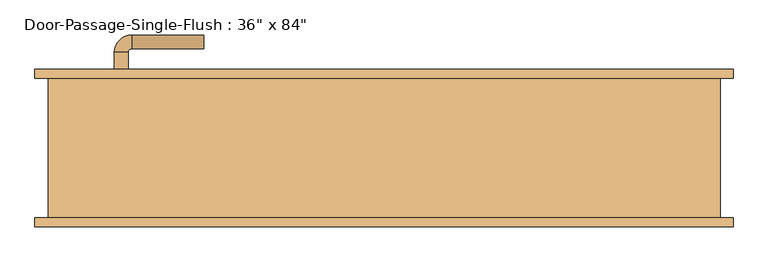
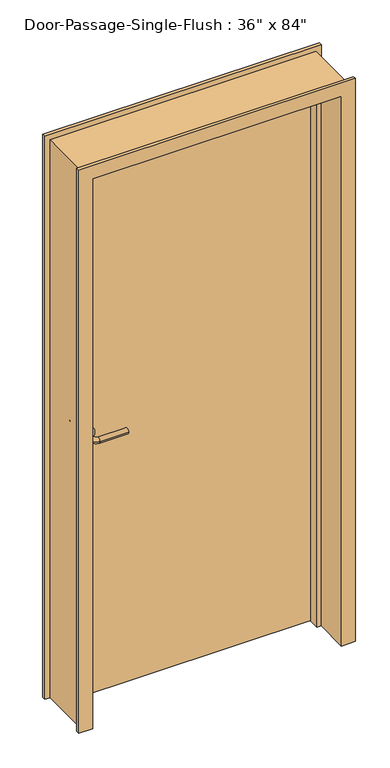
"""IFC4 building model written with IfcOpenShell, lengths in millimetres: door geometry."""

from ifc_helpers import new_model, si_unit, point, frame, frame_2d, origin, origin_with_axes, place, context, project, spatial, polyline, circle_curve, ellipse_curve, trimmed, segment, composite_curve, outline, extrude, faceted_brep, source, transform, mapped, element, save
from ifc_brep_helpers import plane_surface, cylinder_surface, revolved_surface, advanced_brep


def door_7e479f3f(model_context):
    return source(origin(), model_context, "Body", "SolidModel", [
        advanced_brep(
        [(-392.190625, 55.5, 1016.0), (-372.190625, 55.5, 1016.0), (-372.190625, 25.5, 1016.0), (-392.190625, 25.5, 1016.0), (-367.190625, 20.5, 1016.0), (-367.190625, 0.5, 1016.0), (-262.190625, 0.5, 1016.0), (-262.190625, 20.5, 1016.0)],
        [
            (0, 1, circle_curve(frame((-382.190625, 55.5, 1016.0), z_axis=(0.0, 1.0, 0.0), x_axis=(1.0, 0.0, 0.0)), 10.0)),
            (1, 0, circle_curve(frame((-382.190625, 55.5, 1016.0), z_axis=(0.0, 1.0, 0.0), x_axis=(1.0, 0.0, 0.0)), 10.0)),
            (1, 2),
            (2, 3, circle_curve(frame((-382.190625, 25.5, 1016.0), z_axis=(0.0, 1.0, 0.0), x_axis=(1.0, 0.0, 0.0)), 10.0)),
            (3, 0),
            (3, 2, circle_curve(frame((-382.190625, 25.5, 1016.0), z_axis=(0.0, 1.0, 0.0), x_axis=(1.0, 0.0, 0.0)), 10.0)),
            (4, 5, circle_curve(frame((-367.190625, 10.5, 1016.0), z_axis=(-1.0, 0.0, 0.0), x_axis=(0.0, 1.0, 0.0)), 10.0)),
            (5, 3, circle_curve(frame((-367.190625, 25.5, 1016.0), z_axis=(0.0, 0.0, -1.0), x_axis=(-1.0, 0.0, 0.0)), 25.0)),
            (2, 4, circle_curve(frame((-367.190625, 25.5, 1016.0), z_axis=(0.0, 0.0, 1.0), x_axis=(-1.0, 0.0, 0.0)), 5.0)),
            (5, 4, circle_curve(frame((-367.190625, 10.5, 1016.0), z_axis=(-1.0, 0.0, 0.0), x_axis=(0.0, 1.0, 0.0)), 10.0)),
            (6, 7, circle_curve(frame((-262.190625, 10.5, 1016.0), z_axis=(1.0, 0.0, 0.0), x_axis=(0.0, 1.0, 0.0)), 10.0)),
            (7, 6, circle_curve(frame((-262.190625, 10.5, 1016.0), z_axis=(1.0, 0.0, 0.0), x_axis=(0.0, 1.0, 0.0)), 10.0)),
            (4, 7),
            (6, 5),
        ],
        [
            plane_surface(frame((-382.190625, 55.5, 1016.0), z_axis=(0.0, 1.0, 0.0), x_axis=(0.0, 0.0, 1.0))),
            cylinder_surface(frame((-382.190625, 55.5, 1016.0), z_axis=(0.0, 1.0, 0.0), x_axis=(1.0, 0.0, 0.0)), 10.0),
            revolved_surface(trimmed(ellipse_curve(frame((-382.190625, 25.5, 1016.0), z_axis=(0.0, -1.0, 0.0), x_axis=(1.0, 0.0, 0.0)), 10.0, 10.0), [point((-392.190625, 25.5, 1016.0))], [point((-372.190625, 25.5, 1016.0))], True, "CARTESIAN"), (-367.190625, 25.5, 1016.0), (0.0, 0.0, -1.0)),
            revolved_surface(trimmed(ellipse_curve(frame((-382.190625, 25.5, 1016.0), z_axis=(0.0, -1.0, 0.0), x_axis=(1.0, 0.0, 0.0)), 10.0, 10.0), [point((-372.190625, 25.5, 1016.0))], [point((-392.190625, 25.5, 1016.0))], True, "CARTESIAN"), (-367.190625, 25.5, 1016.0), (0.0, 0.0, -1.0)),
            plane_surface(frame((-262.190625, 10.5, 1016.0), z_axis=(1.0, 0.0, 0.0), x_axis=(0.0, 0.0, 1.0))),
            cylinder_surface(frame((-367.190625, 10.5, 1016.0), z_axis=(-1.0, 0.0, 0.0), x_axis=(0.0, 1.0, 0.0)), 10.0),
        ],
        [
            (0, [[1, 2]]),
            (1, [[3, 4, 5, -2]]),
            (1, [[-5, 6, -3, -1]]),
            (2, [[7, 8, -4, 9]]),
            (3, [[10, -9, -6, -8]]),
            (4, [[11, 12]]),
            (5, [[13, -11, 14, -7]]),
            (5, [[-14, -12, -13, -10]]),
        ],
    ),
        extrude(outline(composite_curve([segment(trimmed(circle_curve(frame_2d((1016.0, -384.690625)), 30.0), [point((1016.0, -414.690625))], [point((1016.0, -354.690625))], False, "CARTESIAN"), True, "CONTINUOUS"), segment(trimmed(circle_curve(frame_2d((1016.0, -384.690625)), 30.0), [point((1016.0, -354.690625))], [point((1016.0, -414.690625))], False, "CARTESIAN"), True, "CONTINUOUS")], self_intersect=False)), frame((0.0, 55.5, 0.0), z_axis=(0.0, 1.0, 0.0), x_axis=(0.0, 0.0, 1.0)), (0.0, 0.0, 1.0), 8.0),
        advanced_brep(
        [(-392.190625, 115.95, 1016.0), (-372.190625, 115.95, 1016.0), (-392.190625, 145.95, 1016.0), (-372.190625, 145.95, 1016.0), (-367.190625, 150.95, 1016.0), (-367.190625, 170.95, 1016.0), (-262.190625, 170.95, 1016.0), (-262.190625, 150.95, 1016.0)],
        [
            (0, 1, circle_curve(frame((-382.190625, 115.95, 1016.0), z_axis=(0.0, -1.0, 0.0), x_axis=(1.0, 0.0, 0.0)), 10.0)),
            (1, 0, circle_curve(frame((-382.190625, 115.95, 1016.0), z_axis=(0.0, -1.0, 0.0), x_axis=(1.0, 0.0, 0.0)), 10.0)),
            (0, 2),
            (2, 3, circle_curve(frame((-382.190625, 145.95, 1016.0), z_axis=(0.0, -1.0, 0.0), x_axis=(1.0, 0.0, 0.0)), 10.0)),
            (3, 1),
            (3, 2, circle_curve(frame((-382.190625, 145.95, 1016.0), z_axis=(0.0, -1.0, 0.0), x_axis=(1.0, 0.0, 0.0)), 10.0)),
            (4, 3, circle_curve(frame((-367.190625, 145.95, 1016.0), z_axis=(0.0, 0.0, 1.0), x_axis=(-1.0, 0.0, 0.0)), 5.0)),
            (2, 5, circle_curve(frame((-367.190625, 145.95, 1016.0), z_axis=(0.0, 0.0, -1.0), x_axis=(-1.0, 0.0, 0.0)), 25.0)),
            (5, 4, circle_curve(frame((-367.190625, 160.95, 1016.0), z_axis=(-1.0, 0.0, 0.0), x_axis=(0.0, -1.0, 0.0)), 10.0)),
            (4, 5, circle_curve(frame((-367.190625, 160.95, 1016.0), z_axis=(-1.0, 0.0, 0.0), x_axis=(0.0, -1.0, 0.0)), 10.0)),
            (6, 7, circle_curve(frame((-262.190625, 160.95, 1016.0), z_axis=(1.0, 0.0, 0.0), x_axis=(0.0, -1.0, 0.0)), 10.0)),
            (7, 6, circle_curve(frame((-262.190625, 160.95, 1016.0), z_axis=(1.0, 0.0, 0.0), x_axis=(0.0, -1.0, 0.0)), 10.0)),
            (5, 6),
            (7, 4),
        ],
        [
            plane_surface(frame((-382.190625, 115.95, 1016.0), z_axis=(0.0, -1.0, 0.0), x_axis=(0.0, 0.0, 1.0))),
            cylinder_surface(frame((-382.190625, 115.95, 1016.0), z_axis=(0.0, -1.0, 0.0), x_axis=(1.0, 0.0, 0.0)), 10.0),
            revolved_surface(trimmed(ellipse_curve(frame((-382.190625, 145.95, 1016.0), z_axis=(0.0, -1.0, 0.0), x_axis=(1.0, 0.0, 0.0)), 10.0, 10.0), [point((-392.190625, 145.95, 1016.0))], [point((-372.190625, 145.95, 1016.0))], True, "CARTESIAN"), (-367.190625, 145.95, 1016.0), (0.0, 0.0, -1.0)),
            revolved_surface(trimmed(ellipse_curve(frame((-382.190625, 145.95, 1016.0), z_axis=(0.0, -1.0, 0.0), x_axis=(1.0, 0.0, 0.0)), 10.0, 10.0), [point((-372.190625, 145.95, 1016.0))], [point((-392.190625, 145.95, 1016.0))], True, "CARTESIAN"), (-367.190625, 145.95, 1016.0), (0.0, 0.0, -1.0)),
            plane_surface(frame((-262.190625, 160.95, 1016.0), z_axis=(1.0, 0.0, 0.0), x_axis=(0.0, 0.0, 1.0))),
            cylinder_surface(frame((-367.190625, 160.95, 1016.0), z_axis=(-1.0, 0.0, 0.0), x_axis=(0.0, -1.0, 0.0)), 10.0),
        ],
        [
            (0, [[1, 2]]),
            (1, [[-1, 3, 4, 5]]),
            (1, [[-2, -5, 6, -3]]),
            (2, [[7, -4, 8, 9]]),
            (3, [[-8, -6, -7, 10]]),
            (4, [[11, 12]]),
            (5, [[-9, 13, -12, 14]]),
            (5, [[-10, -14, -11, -13]]),
        ],
    ),
        extrude(outline(composite_curve([segment(trimmed(circle_curve(frame_2d((1016.0, -384.690625)), 30.0), [point((1016.0, -414.690625))], [point((1016.0, -354.690625))], False, "CARTESIAN"), True, "CONTINUOUS"), segment(trimmed(circle_curve(frame_2d((1016.0, -384.690625)), 30.0), [point((1016.0, -354.690625))], [point((1016.0, -414.690625))], False, "CARTESIAN"), True, "CONTINUOUS")], self_intersect=False)), frame((0.0, 107.95, 0.0), z_axis=(0.0, 1.0, 0.0), x_axis=(0.0, 0.0, 1.0)), (0.0, 0.0, 1.0), 8.0),
        faceted_brep([(457.2, 120.65, 0.0), (508.0, 120.65, 0.0), (508.0, 107.95, 0.0), (488.95, 107.95, 0.0), (488.95, -95.25, 0.0), (508.0, -95.25, 0.0), (508.0, -107.95, 0.0), (457.2, -107.95, 0.0), (457.2, 20.6375, 0.0), (441.325, 20.6375, 0.0), (441.325, 58.7375, 0.0), (457.2, 58.7375, 0.0), (457.2, 120.65, 2133.6), (-457.2, 120.65, 2133.6), (-457.2, 120.65, 0.0), (-508.0, 120.65, 0.0), (-508.0, 120.65, 2184.4), (508.0, 120.65, 2184.4), (508.0, 107.95, 2184.4), (-508.0, 107.95, 2184.4), (-508.0, 107.95, 0.0), (-488.95, 107.95, 0.0), (-488.95, 107.95, 2165.35), (488.95, 107.95, 2165.35), (488.95, -95.25, 2165.35), (-488.95, -95.25, 2165.35), (-488.95, -95.25, 0.0), (-508.0, -95.25, 0.0), (-508.0, -95.25, 2184.4), (508.0, -95.25, 2184.4), (508.0, -107.95, 2184.4), (-508.0, -107.95, 2184.4), (-508.0, -107.95, 0.0), (-457.2, -107.95, 0.0), (-457.2, -107.95, 2133.6), (457.2, -107.95, 2133.6), (457.2, 20.6375, 2133.6), (-457.2, 20.6375, 2133.6), (-457.2, 20.6375, 0.0), (-441.325, 20.6375, 0.0), (-441.325, 20.6375, 2117.725), (441.325, 20.6375, 2117.725), (441.325, 58.7375, 2117.725), (-441.325, 58.7375, 2117.725), (-441.325, 58.7375, 0.0), (-457.2, 58.7375, 0.0), (-457.2, 58.7375, 2133.6), (457.2, 58.7375, 2133.6)], [[[0, 1, 2, 3, 4, 5, 6, 7, 8, 9, 10, 11]], [[1, 0, 12, 13, 14, 15, 16, 17]], [[2, 1, 17, 18]], [[3, 2, 18, 19, 20, 21, 22, 23]], [[4, 3, 23, 24]], [[5, 4, 24, 25, 26, 27, 28, 29]], [[6, 5, 29, 30]], [[7, 6, 30, 31, 32, 33, 34, 35]], [[8, 7, 35, 36]], [[9, 8, 36, 37, 38, 39, 40, 41]], [[10, 9, 41, 42]], [[11, 10, 42, 43, 44, 45, 46, 47]], [[0, 11, 47, 12]], [[18, 17, 16, 19]], [[24, 23, 22, 25]], [[30, 29, 28, 31]], [[36, 35, 34, 37]], [[42, 41, 40, 43]], [[12, 47, 46, 13]], [[14, 45, 44, 39, 38, 33, 32, 27, 26, 21, 20, 15]], [[19, 16, 15, 20]], [[25, 22, 21, 26]], [[31, 28, 27, 32]], [[37, 34, 33, 38]], [[43, 40, 39, 44]], [[13, 46, 45, 14]]]),
        extrude(outline(polyline([(457.2, 63.5), (-457.2, 63.5), (-457.2, 107.95), (457.2, 107.95), (457.2, 63.5)])), origin_with_axes(), (0.0, 0.0, 1.0), 2133.6),
    ])


if __name__ == "__main__":
    model = new_model("IFC4")
    model_context = context("Model", 3, world=origin())
    ifc_project = project(units=[si_unit("LENGTHUNIT", "METRE", prefix="MILLI")], contexts=[model_context])
    site = spatial("IfcSite", under=ifc_project)
    building = spatial("IfcBuilding", under=site)
    placement = place(None, origin())
    door_shape = door_7e479f3f(model_context)
    element("IfcDoor", 1, ObjectType="Door-Passage-Single-Flush : 36\" x 84\"", at=placement, inside=building, context=model_context, shape_type="MappedRepresentation", body=[
        mapped(door_shape, transform((0.0, 0.0, 0.0), x_axis=(1.0, 0.0, 0.0), y_axis=(0.0, 1.0, 0.0), z_axis=(0.0, 0.0, 1.0))),
    ])
    save(model, "model.ifc")

# Revit data of these elements
# Type "Door-Passage-Single-Flush : 36\" x 84\""
#   Type Mark = "19"
#   Fire Rating = "--"
#   Assembly Code = "B2030200"
#   Analytic Construction = "Wooden"
#   Thickness = 0' - 1 3/4"
#   Thermal Resistance (R) = 2.5876 (h·ft²·°F)/BTU
#   Swing Angle [instance default] = 90.00°
#   Strike Height = 3' - 4"
#   Rough Width [instance default] = 3' - 4"
#   Rough Height [instance default] = 7' - 4"
#   MF Opening Height [instance default] = 0' - 4"
#   MF Opening Width [instance default] = 0' - 4"
#   Inset Calculate [instance default] = 0' - 4"
#   Masonry Inset [instance default] = 0' - 1"
#   Height = 7' - 0"
#   Width = 3' - 0"
#   Heat Transfer Coefficient (U) = 0.3865 BTU/(h·ft²·°F)
#   Masonry Frame Depth = 0' - 5 3/4"
#   Masonry Frame [instance default] = yes
#   Function = 1
#   Dry Wall Frame [instance default] = no
#   Panel Material = Wood - Birch
#   Frame Material = Metal - Paint Finish - Grey
#   Door Handle Material = Aluminum
#   Visual Light Transmittance = 0
#   Solar Heat Gain Coefficient = 0
#   Wall Closure = (empty or 0)
# Element 1 (IfcDoor, "Door-Passage-Single-Flush : 36\" x 84\"")
#   Rough Width = 3' - 2 1/2"
#   Rough Height = 7' - 1 1/4"
#   MF Opening Height = 0' - 1 1/4"
#   MF Opening Width = 0' - 2 1/2"
#   Inset Calculate = 0' - 3"
#   Masonry Frame = no
#   Dry Wall Frame = yes
#   Materials on its faces: "Metal - Paint Finish - Grey", "Aluminum", "Wood - Birch"
# Materials
#   "Wood - Birch": class "Wood", colour RGB 166 116 52, transparency 0, Cost = 0
#   "Metal - Paint Finish - Grey": class "Paint", colour RGB 104 104 104, transparency 0, Cost = 0
#   "Aluminum": class "Metal", colour RGB 247 247 247, transparency 0, Description = "Aluminum 6061", Cost = 0
